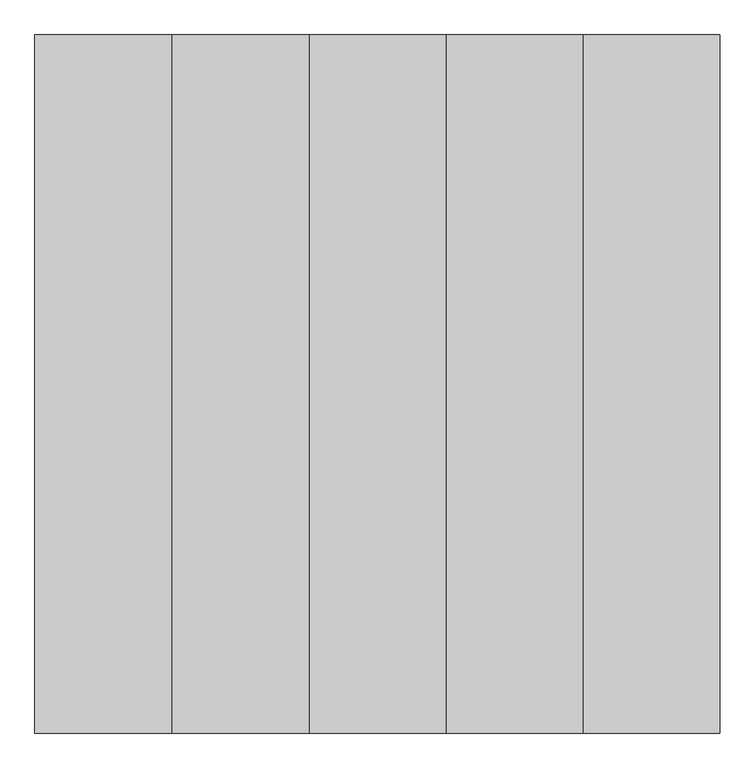
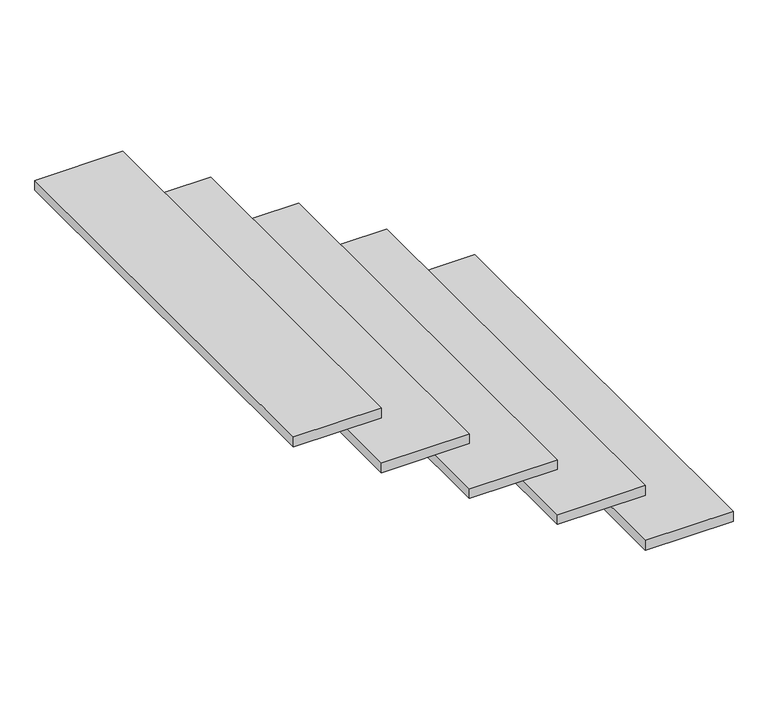
"""IFC4 building model written with IfcOpenShell, lengths in millimetres: stair flight geometry."""

from ifc_helpers import new_model, si_unit, frame, origin, place, context, project, spatial, polyline, outline, extrude, source, transform, mapped, element, save


def stair_flight_4e27faa5(model_context):
    return source(origin(), model_context, "Body", "SweptSolid", [
        extrude(outline(polyline([(47808.2332408, 6860.0306666), (47808.2332408, 8235.0306666), (48078.2332408, 8235.0306666), (48078.2332408, 6860.0306666), (47808.2332408, 6860.0306666)])), frame((0.0, 0.0, 296.5714286), z_axis=(0.0, 0.0, 1.0), x_axis=(1.0, 0.0, 0.0)), (0.0, 0.0, 1.0), 32.0),
        extrude(outline(polyline([(47538.2332408, 6860.0306666), (47538.2332408, 8235.0306666), (47808.2332408, 8235.0306666), (47808.2332408, 6860.0306666), (47538.2332408, 6860.0306666)])), frame((0.0, 0.0, 475.1428571), z_axis=(0.0, 0.0, 1.0), x_axis=(1.0, 0.0, 0.0)), (0.0, 0.0, 1.0), 32.0),
        extrude(outline(polyline([(47268.2332408, 6860.0306666), (47268.2332408, 8235.0306666), (47538.2332408, 8235.0306666), (47538.2332408, 6860.0306666), (47268.2332408, 6860.0306666)])), frame((0.0, 0.0, 653.7142857), z_axis=(0.0, 0.0, 1.0), x_axis=(1.0, 0.0, 0.0)), (0.0, 0.0, 1.0), 32.0),
        extrude(outline(polyline([(46998.2332408, 6860.0306666), (46998.2332408, 8235.0306666), (47268.2332408, 8235.0306666), (47268.2332408, 6860.0306666), (46998.2332408, 6860.0306666)])), frame((0.0, 0.0, 832.2857143), z_axis=(0.0, 0.0, 1.0), x_axis=(1.0, 0.0, 0.0)), (0.0, 0.0, 1.0), 32.0),
        extrude(outline(polyline([(46728.2332408, 6860.0306666), (46728.2332408, 8235.0306666), (46998.2332408, 8235.0306666), (46998.2332408, 6860.0306666), (46728.2332408, 6860.0306666)])), frame((0.0, 0.0, 1010.8571429), z_axis=(0.0, 0.0, 1.0), x_axis=(1.0, 0.0, 0.0)), (0.0, 0.0, 1.0), 32.0),
    ])


if __name__ == "__main__":
    model = new_model("IFC4")
    model_context = context("Model", 3, world=origin())
    ifc_project = project(units=[si_unit("LENGTHUNIT", "METRE", prefix="MILLI")], contexts=[model_context])
    site = spatial("IfcSite", under=ifc_project)
    building = spatial("IfcBuilding", under=site)
    placement = place(None, origin())
    stair_flight_shape = stair_flight_4e27faa5(model_context)
    element("IfcStairFlight", 1, at=placement, inside=building, context=model_context, shape_type="MappedRepresentation", body=[
        mapped(stair_flight_shape, transform((0.0, 0.0, 0.0), x_axis=(1.0, 0.0, 0.0), y_axis=(0.0, 1.0, 0.0), z_axis=(0.0, 0.0, 1.0))),
    ])
    save(model, "model.ifc")
